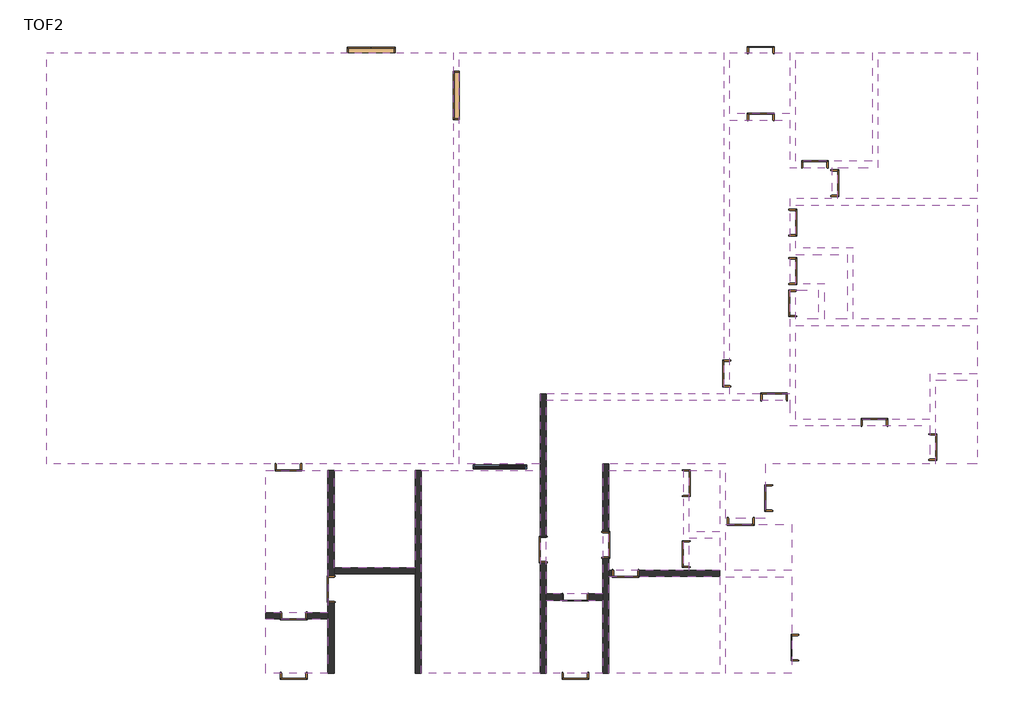
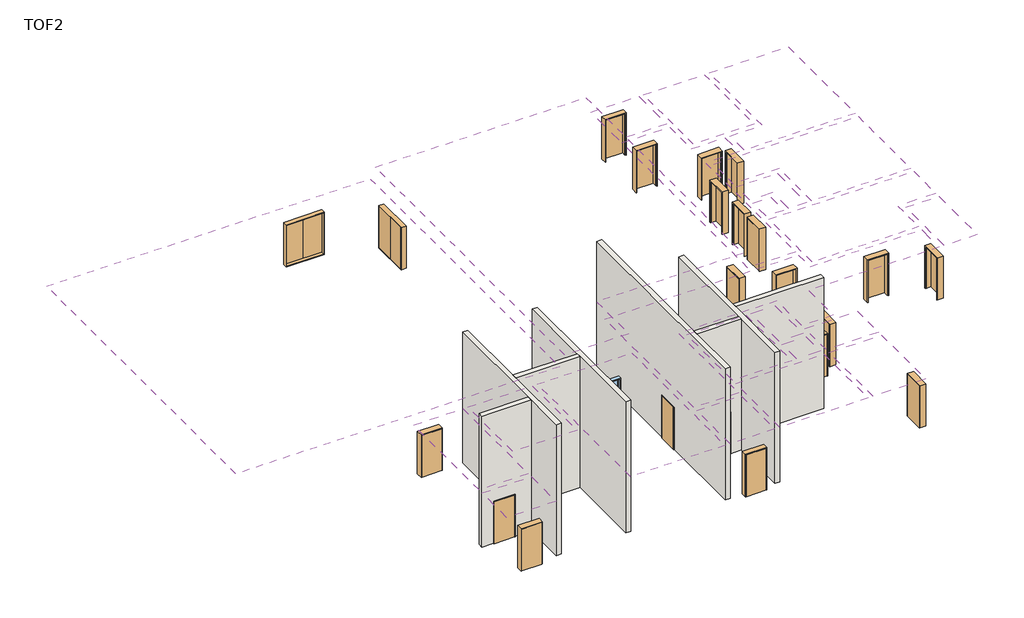
# One storey: 27 doors, 23 coverings, 8 walls, 1 window.
# Revit data of these elements (continued)
# Room at (30337.5, 2458.271) mm, phase "New Construction", upper level "TOC", upper offset 2000 mm, lower offset -2000 mm (continued)
#   H_Ceiling Finish Style Name = "Acrylic Emulsion Paint"
#   H_Ceiling Base Material = "Concrete Slab / Fair Faced Concrete"
#   H_Ceiling-Base Material-1 = "(Concrete Slab)"
#   H_Ceiling-Base Material-2 = ""
#   H_Ceiling-Base Material-3 = ""
#   H_Ceiling-Base Material-4 = ""
#   H_Ceiling-Base Material-5 = ""
#   H_Ceiling Finish-1 = "Acrylic Emulsion Paint"
#   H_Ceiling Finish-2 = ""
#   H_Ceiling Finish Remark = "SACE"
#   Floor Finish Style No = F34A
#   Skirt Finish Style No = B35
#   Wall Finish Style No = W03A
#   Ceiling Finish Style No = C01
# Room at (30407.5, 6398.271) mm, phase "New Construction", upper level "TOC", upper offset 2000 mm, lower offset -2000 mm
#   Comments = ""
#   Number = "113"
#   Name = "STORE"
#   H_Floor Finish Style Name = "Vinyl Tile"
#   H_Floor Base Material = "Concrete Slab / Steel Trowel Finish"
#   H_Wall-Base Material-1 = "Masonry Wall"
#   H_Skirt Finish Style Name = "Coved Vinyl Tile"
#   H_Wall-Base Material-2 = ""
#   H_Wall-Base Material-3 = "Plastering"
#   H_Floor-Base Material-1 = "Concrete Slab"
#   H_Floor-Base Material-2 = "Steel Trowel Finish"
#   H_Floor-Base Material-3 = ""
#   H_Floor-Base Material-4 = ""
#   H_Floor-Base Material-5 = "Vinyl Tile"
#   H_Floor Finish-1 = "Vinyl Tile"
#   H_Floor Finish-2 = ""
#   H_Floor Finish Remark = ""
#   H_Skirt Base Material = "Same as Wall"
#   H_Skirt-Base Material-1 = ""
#   H_Skirt-Base Material-2 = ""
#   H_Skirt-Base Material-3 = ""
#   H_Skirt-Base Material-4 = ""
#   H_Skirt-Base Material-5 = ""
#   H_Skirt Finish-1 = "Vinyl Tile"
#   H_Skirt Finish-2 = ""
#   H_Skirt Finish Remark = "Vinyl Tile = PVC Tile (polyvinyl chloride)"
#   H_Wall Finish Style Name = "Acrylic Emulsion Paint"
#   H_Wall Base Material = "Masonry Wall / Cement Plaster"
#   H_Wall-Base Material-4 = ""
#   H_Wall-Base Material-5 = ""
#   H_Wall Finish-1 = "Acrylic Emulsion Paint"
#   H_Wall Finish-2 = ""
#   H_Wall Finish Remark = "T13 Plaster"
#   H_Ceiling Finish Style Name = "Suspended Acoustic Tiled Ceiling (M-Bar)"
#   H_Ceiling Base Material = "Concrete Slab / Fair Faced Concrete"
#   H_Ceiling-Base Material-1 = "(Concrete Slab)"
#   H_Ceiling-Base Material-2 = "(Fair Faced Concrete)"
#   H_Ceiling-Base Material-3 = ""
#   H_Ceiling-Base Material-4 = ""
#   H_Ceiling-Base Material-5 = "Acoustic Tiled Ceiling System (M-Bar)"
#   H_Ceiling Finish-1 = "Acoustic Tiled Ceiling System (M-Bar)"
#   H_Ceiling Finish-2 = ""
#   H_Ceiling Finish Remark = ""
#   Floor Finish Style No = F34A
#   Skirt Finish Style No = B35
#   Wall Finish Style No = W01B
#   Ceiling Finish Style No = C95A
# Room at (27507.5, 1620.771) mm, phase "New Construction", upper level "TOC", upper offset 2000 mm, lower offset -2000 mm
#   Comments = ""
#   Number = "117"
#   Name = "AIR LOCK"
#   H_Floor Finish Style Name = "Vinyl Tile"
#   H_Floor Base Material = "Concrete Slab / Steel Trowel Finish"
#   H_Wall-Base Material-1 = "Masonry Wall"
#   H_Skirt Finish Style Name = "Coved Vinyl Tile"
#   H_Wall-Base Material-2 = ""
#   H_Wall-Base Material-3 = "Plastering"
#   H_Floor-Base Material-1 = "Concrete Slab"
#   H_Floor-Base Material-2 = "Steel Trowel Finish"
#   H_Floor-Base Material-3 = ""
#   H_Floor-Base Material-4 = ""
#   H_Floor-Base Material-5 = "Vinyl Tile"
#   H_Floor Finish-1 = "Vinyl Tile"
#   H_Floor Finish-2 = ""
#   H_Floor Finish Remark = ""
#   H_Skirt Base Material = "Same as Wall"
#   H_Skirt-Base Material-1 = ""
#   H_Skirt-Base Material-2 = ""
#   H_Skirt-Base Material-3 = ""
#   H_Skirt-Base Material-4 = ""
#   H_Skirt-Base Material-5 = ""
#   H_Skirt Finish-1 = "Vinyl Tile"
#   H_Skirt Finish-2 = ""
#   H_Skirt Finish Remark = "Vinyl Tile = PVC Tile (polyvinyl chloride)"
#   H_Wall Finish Style Name = "Acrylic Emulsion Paint"
#   H_Wall Base Material = "Masonry Wall / Cement Plaster"
#   H_Wall-Base Material-4 = ""
#   H_Wall-Base Material-5 = ""
#   H_Wall Finish-1 = "Acrylic Emulsion Paint"
#   H_Wall Finish-2 = ""
#   H_Wall Finish Remark = "T13 Plaster"
#   H_Ceiling Finish Style Name = "Suspended Acoustic Tiled Ceiling (M-Bar)"
#   H_Ceiling Base Material = "Concrete Slab / Fair Faced Concrete"
#   H_Ceiling-Base Material-1 = "(Concrete Slab)"
#   H_Ceiling-Base Material-2 = "(Fair Faced Concrete)"
#   H_Ceiling-Base Material-3 = ""
#   H_Ceiling-Base Material-4 = ""
#   H_Ceiling-Base Material-5 = "Acoustic Tiled Ceiling System (M-Bar)"
#   H_Ceiling Finish-1 = "Acoustic Tiled Ceiling System (M-Bar)"
#   H_Ceiling Finish-2 = ""
#   H_Ceiling Finish Remark = ""
#   Floor Finish Style No = F34A
#   Skirt Finish Style No = B35
#   Wall Finish Style No = W01B
#   Ceiling Finish Style No = C95A
# Room at (27507.5, 5560.771) mm, phase "New Construction", upper level "TOC", upper offset 2000 mm, lower offset -2000 mm
#   Comments = ""
#   Number = "116"
#   Name = "CORRIDOR"
#   H_Floor Finish Style Name = "Vinyl Tile"
#   H_Floor Base Material = "Concrete Slab / Steel Trowel Finish"
#   H_Wall-Base Material-1 = "Masonry Wall"
#   H_Skirt Finish Style Name = "Coved Vinyl Tile"
#   H_Wall-Base Material-2 = ""
#   H_Wall-Base Material-3 = "Plastering"
#   H_Floor-Base Material-1 = "Concrete Slab"
#   H_Floor-Base Material-2 = "Steel Trowel Finish"
#   H_Floor-Base Material-3 = ""
#   H_Floor-Base Material-4 = ""
#   H_Floor-Base Material-5 = "Vinyl Tile"
#   H_Floor Finish-1 = "Vinyl Tile"
#   H_Floor Finish-2 = ""
#   H_Floor Finish Remark = ""
#   H_Skirt Base Material = "Same as Wall"
#   H_Skirt-Base Material-1 = ""
#   H_Skirt-Base Material-2 = ""
#   H_Skirt-Base Material-3 = ""
#   H_Skirt-Base Material-4 = ""
#   H_Skirt-Base Material-5 = ""
#   H_Skirt Finish-1 = "Vinyl Tile"
#   H_Skirt Finish-2 = ""
#   H_Skirt Finish Remark = "Vinyl Tile = PVC Tile (polyvinyl chloride)"
#   H_Wall Finish Style Name = "Acrylic Emulsion Paint"
#   H_Wall Base Material = "Masonry Wall / Cement Plaster"
#   H_Wall-Base Material-4 = ""
#   H_Wall-Base Material-5 = ""
#   H_Wall Finish-1 = "Acrylic Emulsion Paint"
#   H_Wall Finish-2 = ""
#   H_Wall Finish Remark = "T13 Plaster"
#   H_Ceiling Finish Style Name = "Suspended Acoustic Tiled Ceiling (M-Bar)"
#   H_Ceiling Base Material = "Concrete Slab / Fair Faced Concrete"
#   H_Ceiling-Base Material-1 = "(Concrete Slab)"
#   H_Ceiling-Base Material-2 = "(Fair Faced Concrete)"
#   H_Ceiling-Base Material-3 = ""
#   H_Ceiling-Base Material-4 = ""
#   H_Ceiling-Base Material-5 = "Acoustic Tiled Ceiling System (M-Bar)"
#   H_Ceiling Finish-1 = "Acoustic Tiled Ceiling System (M-Bar)"
#   H_Ceiling Finish-2 = ""
#   H_Ceiling Finish Remark = ""
#   Floor Finish Style No = F34A
#   Skirt Finish Style No = B35
#   Wall Finish Style No = W01B
#   Ceiling Finish Style No = C95A
# Room at (43950, 7179.173) mm, phase "New Construction", upper level "TOC", upper offset 2000 mm, lower offset -2000 mm
#   Comments = ""
#   Number = "120"
#   Name = "CORRIDOR"
#   H_Floor Finish Style Name = "Vinyl Tile"
#   H_Floor Base Material = "Concrete Slab / Steel Trowel Finish"
#   H_Wall-Base Material-1 = "Masonry Wall"
#   H_Skirt Finish Style Name = "Coved Vinyl Tile"
#   H_Wall-Base Material-2 = ""
#   H_Wall-Base Material-3 = "Plastering"
#   H_Floor-Base Material-1 = "Concrete Slab"
#   H_Floor-Base Material-2 = "Steel Trowel Finish"
#   H_Floor-Base Material-3 = ""
#   H_Floor-Base Material-4 = ""
#   H_Floor-Base Material-5 = "Vinyl Tile"
#   H_Floor Finish-1 = "Vinyl Tile"
#   H_Floor Finish-2 = ""
#   H_Floor Finish Remark = ""
#   H_Skirt Base Material = "Same as Wall"
#   H_Skirt-Base Material-1 = ""
#   H_Skirt-Base Material-2 = ""
#   H_Skirt-Base Material-3 = ""
#   H_Skirt-Base Material-4 = ""
#   H_Skirt-Base Material-5 = ""
#   H_Skirt Finish-1 = "Vinyl Tile"
#   H_Skirt Finish-2 = ""
#   H_Skirt Finish Remark = "Vinyl Tile = PVC Tile (polyvinyl chloride)"
#   H_Wall Finish Style Name = "Acrylic Emulsion Paint"
#   H_Wall Base Material = "Masonry Wall / Cement Plaster"
#   H_Wall-Base Material-4 = ""
#   H_Wall-Base Material-5 = ""
#   H_Wall Finish-1 = "Acrylic Emulsion Paint"
#   H_Wall Finish-2 = ""
#   H_Wall Finish Remark = "T13 Plaster"
#   H_Ceiling Finish Style Name = "Suspended Acoustic Tiled Ceiling (M-Bar)"
#   H_Ceiling Base Material = "Concrete Slab / Fair Faced Concrete"
#   H_Ceiling-Base Material-1 = "(Concrete Slab)"
#   H_Ceiling-Base Material-2 = "(Fair Faced Concrete)"
#   H_Ceiling-Base Material-3 = ""
#   H_Ceiling-Base Material-4 = ""
#   H_Ceiling-Base Material-5 = "Acoustic Tiled Ceiling System (M-Bar)"
#   H_Ceiling Finish-1 = "Acoustic Tiled Ceiling System (M-Bar)"
#   H_Ceiling Finish-2 = ""
#   H_Ceiling Finish Remark = ""
#   Floor Finish Style No = F34A
#   Skirt Finish Style No = B35
#   Wall Finish Style No = W01B
#   Ceiling Finish Style No = C95A
# Room at (37875, 1969.173) mm, phase "New Construction", upper level "TOC", upper offset 2000 mm, lower offset -2000 mm
#   Comments = ""
#   Number = "119"
#   Name = "AIR LOCK"
#   H_Floor Finish Style Name = "Vinyl Tile"
#   H_Floor Base Material = "Concrete Slab / Steel Trowel Finish"
#   H_Wall-Base Material-1 = "Masonry Wall"
#   H_Skirt Finish Style Name = "Coved Vinyl Tile"
#   H_Wall-Base Material-2 = ""
#   H_Wall-Base Material-3 = "Plastering"
#   H_Floor-Base Material-1 = "Concrete Slab"
#   H_Floor-Base Material-2 = "Steel Trowel Finish"
#   H_Floor-Base Material-3 = ""
#   H_Floor-Base Material-4 = ""
#   H_Floor-Base Material-5 = "Vinyl Tile"
#   H_Floor Finish-1 = "Vinyl Tile"
#   H_Floor Finish-2 = ""
#   H_Floor Finish Remark = ""
#   H_Skirt Base Material = "Same as Wall"
#   H_Skirt-Base Material-1 = ""
#   H_Skirt-Base Material-2 = ""
#   H_Skirt-Base Material-3 = ""
#   H_Skirt-Base Material-4 = ""
#   H_Skirt-Base Material-5 = ""
#   H_Skirt Finish-1 = "Vinyl Tile"
#   H_Skirt Finish-2 = ""
#   H_Skirt Finish Remark = "Vinyl Tile = PVC Tile (polyvinyl chloride)"
#   H_Wall Finish Style Name = "Acrylic Emulsion Paint"
#   H_Wall Base Material = "Masonry Wall / Cement Plaster"
#   H_Wall-Base Material-4 = ""
#   H_Wall-Base Material-5 = ""
#   H_Wall Finish-1 = "Acrylic Emulsion Paint"
#   H_Wall Finish-2 = ""
#   H_Wall Finish Remark = "T13 Plaster"
#   H_Ceiling Finish Style Name = "Suspended Acoustic Tiled Ceiling (M-Bar)"
#   H_Ceiling Base Material = "Concrete Slab / Fair Faced Concrete"
#   H_Ceiling-Base Material-1 = "(Concrete Slab)"
#   H_Ceiling-Base Material-2 = "(Fair Faced Concrete)"
#   H_Ceiling-Base Material-3 = ""
#   H_Ceiling-Base Material-4 = ""
#   H_Ceiling-Base Material-5 = "Acoustic Tiled Ceiling System (M-Bar)"
#   H_Ceiling Finish-1 = "Acoustic Tiled Ceiling System (M-Bar)"
#   H_Ceiling Finish-2 = ""
#   H_Ceiling Finish Remark = ""
#   Floor Finish Style No = F34A
#   Skirt Finish Style No = B35
#   Wall Finish Style No = W01B
#   Ceiling Finish Style No = C95A
